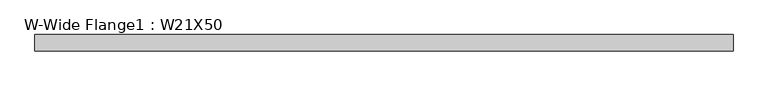
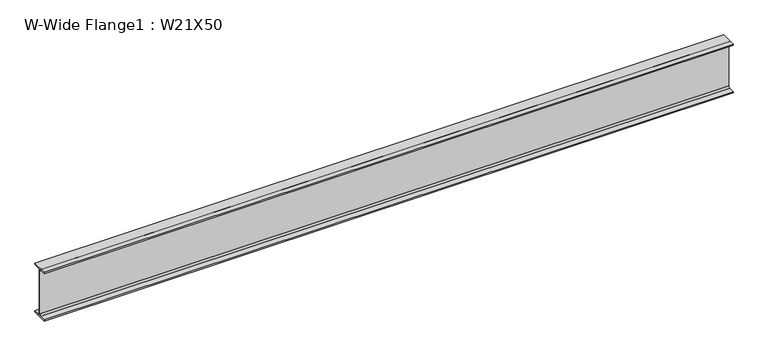
"""IFC4 building model written with IfcOpenShell, lengths in millimetres: beam geometry, W-Wide Flange1 : W21X50."""

from ifc_helpers import new_model, si_unit, point, frame, frame_2d, origin, place, context, project, spatial, polyline, circle_curve, trimmed, segment, composite_curve, outline, extrude, source, transform, mapped, element, save


def w_wide_flange1_w21x50_e64ade31(model_context):
    return source(origin(), model_context, "Body", "SweptSolid", [
        extrude(outline(composite_curve([segment(polyline([(82.931, -250.571), (82.931, -264.16), (-82.931, -264.16), (-82.931, -250.571), (-22.987, -250.571)]), True, "CONTINUOUS"), segment(trimmed(circle_curve(frame_2d((-22.987, -232.41)), 18.161), [point((-22.987, -250.571))], [point((-4.826, -232.41))], True, "CARTESIAN"), True, "CONTINUOUS"), segment(polyline([(-4.826, -232.41), (-4.826, 232.41)]), True, "CONTINUOUS"), segment(trimmed(circle_curve(frame_2d((-22.987, 232.41)), 18.161), [point((-4.826, 232.41))], [point((-22.987, 250.571))], True, "CARTESIAN"), True, "CONTINUOUS"), segment(polyline([(-22.987, 250.571), (-82.931, 250.571), (-82.931, 264.16), (82.931, 264.16), (82.931, 250.571), (22.987, 250.571)]), True, "CONTINUOUS"), segment(trimmed(circle_curve(frame_2d((22.987, 232.41)), 18.161), [point((22.987, 250.571))], [point((4.826, 232.41))], True, "CARTESIAN"), True, "CONTINUOUS"), segment(polyline([(4.826, 232.41), (4.826, -232.41)]), True, "CONTINUOUS"), segment(trimmed(circle_curve(frame_2d((22.987, -232.41)), 18.161), [point((4.826, -232.41))], [point((22.987, -250.571))], True, "CARTESIAN"), True, "CONTINUOUS"), segment(polyline([(22.987, -250.571), (82.931, -250.571)]), True, "CONTINUOUS")], self_intersect=False)), frame((-3529.877, 0.0, 0.0), z_axis=(1.0, 0.0, 0.0), x_axis=(0.0, 1.0, 0.0)), (0.0, 0.0, 1.0), 7059.754),
    ])


if __name__ == "__main__":
    model = new_model("IFC4")
    model_context = context("Model", 3, world=origin())
    ifc_project = project(units=[si_unit("LENGTHUNIT", "METRE", prefix="MILLI")], contexts=[model_context])
    site = spatial("IfcSite", under=ifc_project)
    building = spatial("IfcBuilding", under=site)
    placement = place(None, origin())
    w_wide_flange1_w21x50_shape = w_wide_flange1_w21x50_e64ade31(model_context)
    element("IfcBeam", 1, ObjectType="W-Wide Flange1 : W21X50", at=placement, inside=building, context=model_context, shape_type="MappedRepresentation", body=[
        mapped(w_wide_flange1_w21x50_shape, transform((0.0, 0.0, 0.0), x_axis=(1.0, 0.0, 0.0), y_axis=(0.0, 1.0, 0.0), z_axis=(0.0, 0.0, 1.0))),
    ])
    save(model, "model.ifc")

# Revit data of these elements
# Type "W-Wide Flange1 : W21X50"
#   Assembly Code = "B10"
#   W = 50
#   Start Extension Calculation [instance default] = 10' - 0"
#   Start Extension [instance default] = -0' - 0 1/2"
#   End Extension Calculation [instance default] = 10' - 0"
#   End Extension [instance default] = -0' - 0 1/2"
#   Length [instance default] = 5' - 0"
#   bf = 0' - 6.53"
#   d = 1' - 8.8"
#   k = 0' - 1 1/4"
#   k2 = 0' - 0.715"
#   tf = 0' - 0.535"
#   tw = 0' - 0.38"
#   A = 0.102083 SF
#   Structural Material [instance default] = Metal - Steel - ASTM A992
# Element 1 (IfcBeam, "W-Wide Flange1 : W21X50")
#   Materials on its faces: "Metal - Steel - ASTM A992"
# Materials
#   "Metal - Steel - ASTM A992": class "Metal", colour RGB 199 199 199, transparency 0
